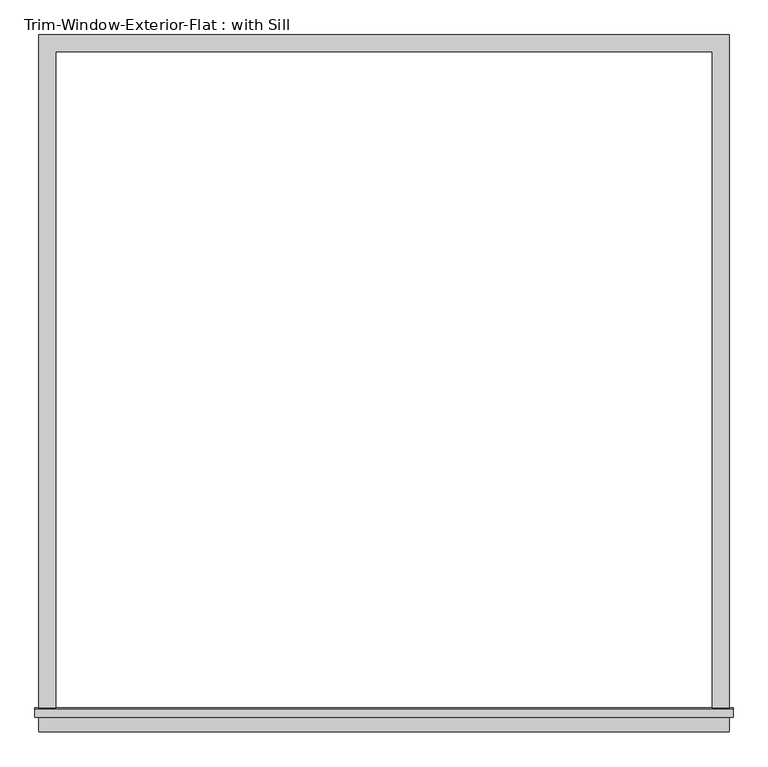
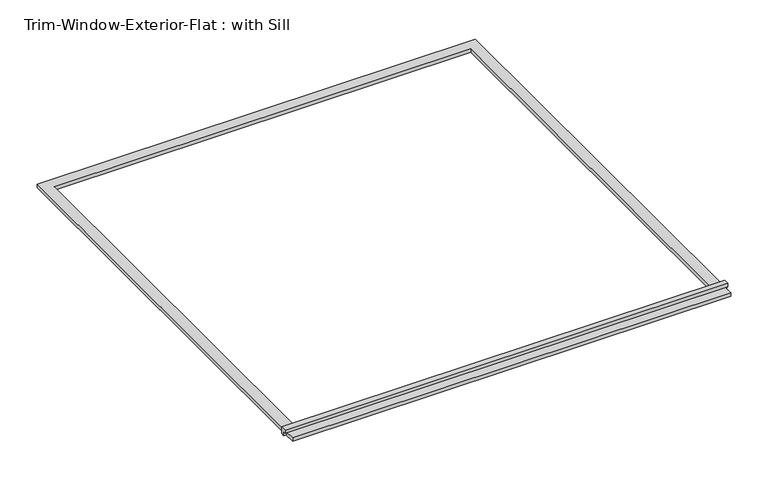
"""IFC4 building model written with IfcOpenShell, lengths in millimetres: proxy geometry, Trim-Window-Exterior-Flat : with Sill."""

from ifc_helpers import new_model, si_unit, frame, origin, origin_with_axes, place, context, project, spatial, polyline, outline, extrude, source, transform, mapped, element, save


def trim_window_exterior_flat_with_sill_95fde1b8(model_context):
    return source(origin(), model_context, "Body", "SweptSolid", [
        extrude(outline(polyline([(1157.15, -2222.1823709), (1157.15, -2279.3323709), (-1157.15, -2279.3323709), (-1157.15, -2222.1823709), (1157.15, -2222.1823709)])), origin_with_axes(), (0.0, 0.0, 1.0), 19.05),
        extrude(outline(polyline([(-2231.75, 38.1), (-2202.4580645, 38.1), (-2200.0, 19.05), (-2200.0, 0.0), (-2222.1823709, 0.0), (-2222.1823709, 19.05), (-2231.75, 19.05), (-2231.75, 38.1)])), frame((-1169.85, 0.0, 0.0), z_axis=(1.0, 0.0, 0.0), x_axis=(0.0, 1.0, 0.0)), (0.0, 0.0, 1.0), 2339.7),
        extrude(outline(polyline([(-1157.15, 57.15), (1157.15, 57.15), (1157.15, -2200.0), (1100.0, -2200.0), (1100.0, 0.0), (-1100.0, 0.0), (-1100.0, -2200.0), (-1157.15, -2200.0), (-1157.15, 57.15)])), origin_with_axes(), (0.0, 0.0, 1.0), 19.05),
    ])


if __name__ == "__main__":
    model = new_model("IFC4")
    model_context = context("Model", 3, world=origin())
    ifc_project = project(units=[si_unit("LENGTHUNIT", "METRE", prefix="MILLI")], contexts=[model_context])
    site = spatial("IfcSite", under=ifc_project)
    building = spatial("IfcBuilding", under=site)
    placement = place(None, origin())
    trim_window_exterior_flat_with_sill_shape = trim_window_exterior_flat_with_sill_95fde1b8(model_context)
    element("IfcBuildingElementProxy", 1, Name="Trim-Window-Exterior-Flat : with Sill", ObjectType="Trim-Window-Exterior-Flat : with Sill", at=placement, inside=building, context=model_context, shape_type="MappedRepresentation", body=[
        mapped(trim_window_exterior_flat_with_sill_shape, transform((0.0, 0.0, 0.0), x_axis=(1.0, 0.0, 0.0), y_axis=(0.0, 1.0, 0.0), z_axis=(0.0, 0.0, 1.0))),
    ])
    save(model, "model.ifc")

# Revit data of these elements
# Type "Trim-Window-Exterior-Flat : with Sill"
#   Trim Width = 0.05715 m
#   Trim Thickness_Picture Frame = 0.03175 m
#   Trim Thickness_with Sill = 0.01905 m
#   Sill Thickness = 0.03175 m
#   Opening Width [instance default] = 0.6096 m
#   Opening Height [instance default] = 0.9144 m
#   Default Elevation = 1.2192 m
#   Sill = yes
#   Picture Frame = no
#   Trim Material [instance default] = none
# Element 1 (IfcBuildingElementProxy, "Trim-Window-Exterior-Flat : with Sill")
#   Opening Width = 2.2 m
#   Opening Height = 2.2 m
#   Trim Material = Clad - White
#   Materials on its faces: "Clad - White"
# Materials
#   "Clad - White": class "Wood", colour RGB 242 242 238, transparency 0, Cost = 0
